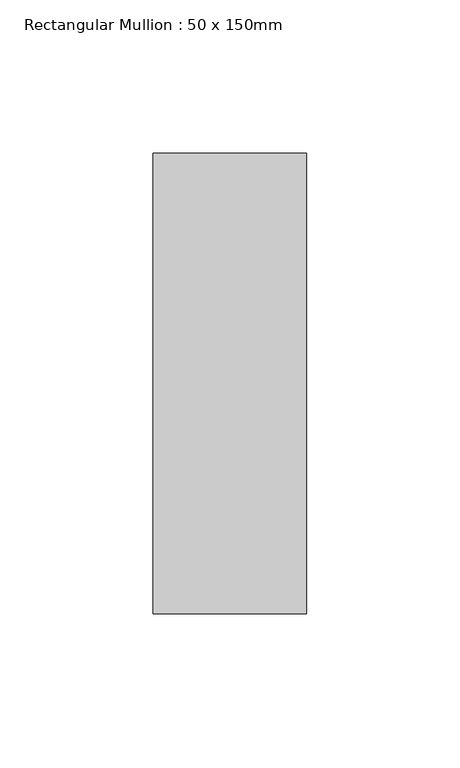
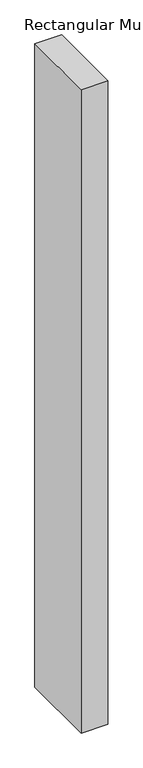
"""IFC4 building model written with IfcOpenShell, lengths in millimetres: member geometry, Rectangular Mullion : 50 x 150mm."""

import ifcopenshell
import ifcopenshell.guid

model = None  # the IFC model being written
_history = None  # IfcOwnerHistory: only IFC2X3 demands one
_inside = {}  # id of a spatial element -> (the spatial element, [elements in it])
_under = {}  # id of a project, library or spatial element -> (it, [spatial elements below it])
_declared = {}  # id of a project -> (the project, [libraries it declares])
_typed = {}  # id of a type object -> (the type object, [elements of that type])
_made_of = {}  # id of a material, layer set ... -> (it, [elements and type objects made of it])


def new_model(schema):
    """Start an empty IFC model of exactly this schema.

    Asked for "IFC4X3", IfcOpenShell would pick the latest addendum, in which some entities
    have other attributes; the version numbers below select the first issue.
    IFC2X3 requires an IfcOwnerHistory on every rooted entity: one is made here for all.
    """
    global model, _history
    if schema == "IFC4X3":
        model = ifcopenshell.file(schema_version=(4, 3, 0, 0))
    else:
        model = ifcopenshell.file(schema=schema)
    _inside.clear()
    _under.clear()
    _declared.clear()
    _typed.clear()
    _made_of.clear()
    _history = None
    if model.schema == "IFC2X3":
        org = make("IfcOrganization", Name="unknown")
        user = make(
            "IfcPersonAndOrganization",
            ThePerson=make("IfcPerson", FamilyName="unknown"),
            TheOrganization=org,
        )
        app = make(
            "IfcApplication",
            ApplicationDeveloper=org,
            Version="unknown",
            ApplicationFullName="unknown",
            ApplicationIdentifier="unknown",
        )
        _history = make(
            "IfcOwnerHistory",
            OwningUser=user,
            OwningApplication=app,
            ChangeAction="ADDED",
            CreationDate=0,
        )
    return model


def make(cls, **values):
    """One entity of the class cls with the attributes given. An attribute that is None is left unset."""
    return model.create_entity(
        cls, **{name: value for name, value in values.items() if value is not None}
    )


def rooted(cls, **values):
    """An entity with a GlobalId (a new one), such as an element, a storey or a relation."""
    return make(cls, GlobalId=ifcopenshell.guid.new(), OwnerHistory=_history, **values)


def si_unit(unit_type, name, prefix=None):
    """IfcSIUnit, for example si_unit("LENGTHUNIT", "METRE", prefix="MILLI")."""
    return make("IfcSIUnit", UnitType=unit_type, Prefix=prefix, Name=name)


def assignment(units):
    """IfcUnitAssignment: the units of a project."""
    return None if units is None else make("IfcUnitAssignment", Units=units)


def point(xyz):
    """IfcCartesianPoint."""
    return None if xyz is None else make("IfcCartesianPoint", Coordinates=xyz)


def direction(xyz):
    """IfcDirection."""
    return None if xyz is None else make("IfcDirection", DirectionRatios=xyz)


def frame(location, z_axis=None, x_axis=None):
    """IfcAxis2Placement3D, a coordinate frame: its origin and axes. An axis left out is left unset."""
    return make(
        "IfcAxis2Placement3D",
        Location=point(location),
        Axis=direction(z_axis),
        RefDirection=direction(x_axis),
    )


def origin():
    """The frame at (0, 0, 0) with its axes left unset."""
    return frame((0.0, 0.0, 0.0))


def place(relative_to, where):
    """IfcLocalPlacement: puts the frame where relative to a parent placement (None: the world)."""
    return make(
        "IfcLocalPlacement", PlacementRelTo=relative_to, RelativePlacement=where
    )


def context(
    kind, dimensions, precision=None, world=None, true_north=None, identifier=None
):
    """IfcGeometricRepresentationContext, for example the 3D "Model" context."""
    return make(
        "IfcGeometricRepresentationContext",
        ContextIdentifier=identifier,
        ContextType=kind,
        CoordinateSpaceDimension=dimensions,
        Precision=precision,
        WorldCoordinateSystem=world,
        TrueNorth=true_north,
    )


def project(units=None, contexts=None):
    """IfcProject with its units and contexts."""
    return rooted(
        "IfcProject",
        Name="project",
        RepresentationContexts=contexts,
        UnitsInContext=assignment(units),
    )


def spatial(cls, under=None, at=None, **own):
    """A site, building, storey or space (cls), placed at a placement, below another one or the project."""
    s = rooted(cls, ObjectPlacement=at, **own)
    if under is not None:
        _under.setdefault(under.id(), (under, []))[1].append(s)
    return s


def polyline(points):
    """IfcPolyline through the points."""
    return make("IfcPolyline", Points=[point(p) for p in points])


def outline(outer, holes=None, kind="AREA"):
    """IfcArbitraryClosedProfileDef: a profile drawn as a closed curve; with holes, ...WithVoids."""
    if holes is None:
        return make("IfcArbitraryClosedProfileDef", ProfileType=kind, OuterCurve=outer)
    return make(
        "IfcArbitraryProfileDefWithVoids",
        ProfileType=kind,
        OuterCurve=outer,
        InnerCurves=holes,
    )


def extrude(swept, where, along, depth):
    """IfcExtrudedAreaSolid: the profile swept, set in the frame where, extruded along a direction by depth."""
    return make(
        "IfcExtrudedAreaSolid",
        SweptArea=swept,
        Position=where,
        ExtrudedDirection=direction(along),
        Depth=depth,
    )


def shape(context_of_items, identifier, shape_type, items):
    """IfcShapeRepresentation: the items that make up one representation, for example the "Body"."""
    return make(
        "IfcShapeRepresentation",
        ContextOfItems=context_of_items,
        RepresentationIdentifier=identifier,
        RepresentationType=shape_type,
        Items=items,
    )


def source(mapping_origin, context_of_items, identifier, shape_type, items):
    """IfcRepresentationMap: a shape defined once, which mapped items show again and again."""
    return make(
        "IfcRepresentationMap",
        MappingOrigin=mapping_origin,
        MappedRepresentation=shape(context_of_items, identifier, shape_type, items),
    )


def transform(
    local_origin,
    x_axis=None,
    y_axis=None,
    z_axis=None,
    scale=None,
    scale2=None,
    scale3=None,
    uniform=True,
):
    """IfcCartesianTransformationOperator3D, or its non-uniform kind. x_axis, y_axis, z_axis: its Axis1, 2, 3."""
    if uniform:
        return make(
            "IfcCartesianTransformationOperator3D",
            Axis1=direction(x_axis),
            Axis2=direction(y_axis),
            LocalOrigin=point(local_origin),
            Scale=scale,
            Axis3=direction(z_axis),
        )
    return make(
        "IfcCartesianTransformationOperator3DnonUniform",
        Axis1=direction(x_axis),
        Axis2=direction(y_axis),
        LocalOrigin=point(local_origin),
        Scale=scale,
        Axis3=direction(z_axis),
        Scale2=scale2,
        Scale3=scale3,
    )


def mapped(mapping_source, mapping_target):
    """IfcMappedItem: shows the shape of a source again, moved by a transform."""
    return make(
        "IfcMappedItem", MappingSource=mapping_source, MappingTarget=mapping_target
    )


def made_of(thing, what):
    """Note that an element or type object is made of a material, layer set ...; save() writes the relation."""
    if what is not None:
        _made_of.setdefault(what.id(), (what, []))[1].append(thing)
    return thing


def element(
    cls,
    number,
    at=None,
    inside=None,
    cuts=None,
    type_object=None,
    material=None,
    context=None,
    identifier="Body",
    shape_type=None,
    held_by="IfcProductDefinitionShape",
    body=None,
    shapes=None,
    **own,
):
    """One element of the class cls, such as IfcWall. Its Tag is "e" and its number.

    at: its placement. inside: the storey or other place that contains it. cuts: it is an
    opening in that element (IfcRelVoidsElement). A single representation is given by context,
    identifier, shape_type and body (its items); several are given by shapes. held_by: the class
    of the entity that holds the representations. save() writes the other relations.
    """
    e = rooted(cls, Tag="e%d" % number, ObjectPlacement=at, **own)
    if body is not None:
        shapes = [shape(context, identifier, shape_type, body)]
    if shapes is not None:
        e.Representation = make(held_by, Representations=shapes)
    if inside is not None:
        _inside.setdefault(inside.id(), (inside, []))[1].append(e)
    if cuts is not None:
        rooted(
            "IfcRelVoidsElement", RelatingBuildingElement=cuts, RelatedOpeningElement=e
        )
    if type_object is not None:
        _typed.setdefault(type_object.id(), (type_object, []))[1].append(e)
    return made_of(e, material)


def aggregate(whole, parts):
    """IfcRelAggregates: a whole, such as a stair, and the parts it consists of."""
    return rooted("IfcRelAggregates", RelatingObject=whole, RelatedObjects=parts)


def save(model, path):
    """Write the relations noted so far, then the file.

    IfcRelAggregates (storeys below a building ...), IfcRelContainedInSpatialStructure (elements
    in a storey), IfcRelDefinesByType, IfcRelAssociatesMaterial and IfcRelDeclares: one each for
    every whole, place, type object, material and project.
    """
    for whole, parts in _under.values():
        aggregate(whole, parts)
    for where, things in _inside.values():
        rooted(
            "IfcRelContainedInSpatialStructure",
            RelatedElements=things,
            RelatingStructure=where,
        )
    for kind, things in _typed.values():
        rooted("IfcRelDefinesByType", RelatedObjects=things, RelatingType=kind)
    for what, things in _made_of.values():
        rooted("IfcRelAssociatesMaterial", RelatedObjects=things, RelatingMaterial=what)
    for by, libraries in _declared.values():
        rooted("IfcRelDeclares", RelatingContext=by, RelatedDefinitions=libraries)
    model.write(path)


def rectangular_mullion_50_x_150mm_345eee08(model_context):
    return source(origin(), model_context, "Body", "SweptSolid", [
        extrude(outline(polyline([(0.0, 75.0), (0.0, -75.0), (-50.0, -75.0), (-50.0, 75.0), (0.0, 75.0)])), frame((0.0, 0.0, -1274.9999998), z_axis=(0.0, 0.0, 1.0), x_axis=(1.0, 0.0, 0.0)), (0.0, 0.0, 1.0), 1274.9999998),
    ])


if __name__ == "__main__":
    model = new_model("IFC4")
    model_context = context("Model", 3, world=origin())
    ifc_project = project(units=[si_unit("LENGTHUNIT", "METRE", prefix="MILLI")], contexts=[model_context])
    site = spatial("IfcSite", under=ifc_project)
    building = spatial("IfcBuilding", under=site)
    placement = place(None, origin())
    rectangular_mullion_50_x_150mm_shape = rectangular_mullion_50_x_150mm_345eee08(model_context)
    element("IfcMember", 1, ObjectType="Rectangular Mullion : 50 x 150mm", at=placement, inside=building, context=model_context, shape_type="MappedRepresentation", body=[
        mapped(rectangular_mullion_50_x_150mm_shape, transform((0.0, 0.0, 0.0), x_axis=(1.0, 0.0, 0.0), y_axis=(0.0, 1.0, 0.0), z_axis=(0.0, 0.0, 1.0))),
    ])
    save(model, "model.ifc")

# Revit data of these elements
# Type "Rectangular Mullion : 50 x 150mm"
#   built-in parameter 1007304 = 0.492126 (stored number, unit not read)
#   built-in parameter 1007301 = 0.082021 (stored number, unit not read)
#   built-in parameter 1007300 = 0.082021 (stored number, unit not read)
# Element 1 (IfcMember, "Rectangular Mullion : 50 x 150mm")
#   Materials on its faces: "Aluminium"
# Materials
#   "Aluminium": class "Metal", colour RGB 247 247 247, transparency 0, Description = "Aluminium 6061", Cost = 0
